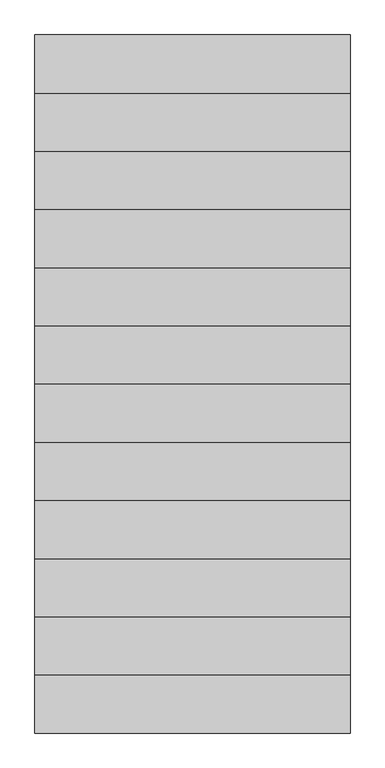
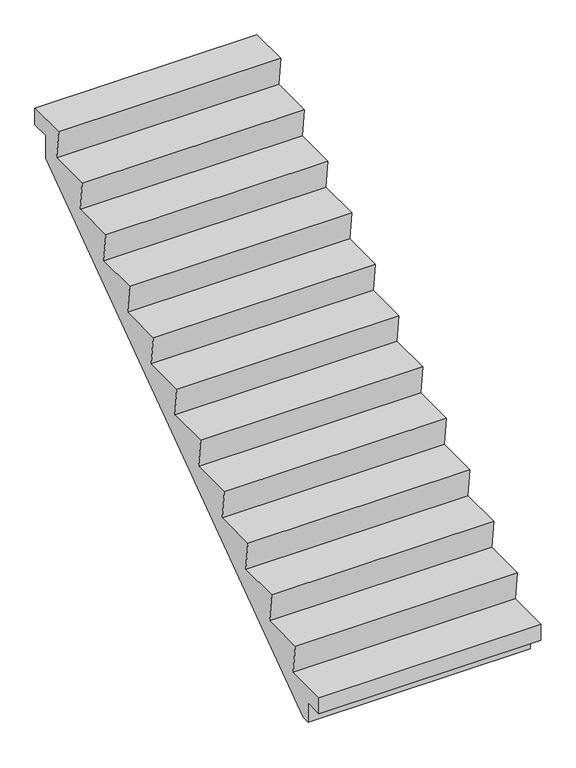
"""IFC4 building model written with IfcOpenShell, lengths in millimetres: stair geometry, NLRS_24_GM_LB_rechte steektrap prefab-AV_gen_rsf : prefab trap_gen__aant=11 b=1200 a=220 o=172.7 zonder bomen."""

from ifc_helpers import new_model, si_unit, frame, origin, place, context, project, spatial, polyline, outline, extrude, source, transform, mapped, element, save


def stair_98d4c19e(model_context):
    return source(origin(), model_context, "Body", "SweptSolid", [
        extrude(outline(polyline([(2400.0, 1900.0), (2640.0, 1900.0), (2640.0, 1800.0), (2530.0, 1800.0), (2530.0, 1658.5925892), (-80.254966, -220.0), (-130.0, -220.0), (-130.0, -100.0), (-240.0, -100.0), (-240.0, 0.0), (20.0, 0.0), (0.0, 172.7272727), (260.0, 172.7272727), (240.0, 345.4545455), (500.0, 345.4545455), (480.0, 518.1818182), (740.0, 518.1818182), (720.0, 690.9090909), (980.0, 690.9090909), (960.0, 863.6363636), (1220.0, 863.6363636), (1200.0, 1036.3636364), (1460.0, 1036.3636364), (1440.0, 1209.0909091), (1700.0, 1209.0909091), (1680.0, 1381.8181818), (1940.0, 1381.8181818), (1920.0, 1554.5454545), (2180.0, 1554.5454545), (2160.0, 1727.2727273), (2420.0, 1727.2727273), (2400.0, 1900.0)])), frame((-650.0, 0.0, 0.0), z_axis=(1.0, 0.0, 0.0), x_axis=(0.0, 1.0, 0.0)), (0.0, 0.0, 1.0), 1300.0),
    ])


if __name__ == "__main__":
    model = new_model("IFC4")
    model_context = context("Model", 3, world=origin())
    ifc_project = project(units=[si_unit("LENGTHUNIT", "METRE", prefix="MILLI")], contexts=[model_context])
    site = spatial("IfcSite", under=ifc_project)
    building = spatial("IfcBuilding", under=site)
    placement = place(None, origin())
    stair_shape = stair_98d4c19e(model_context)
    element("IfcStair", 1, ObjectType="NLRS_24_GM_LB_rechte steektrap prefab-AV_gen_rsf : prefab trap_gen__aant=11 b=1200 a=220 o=172.7 zonder bomen", at=placement, inside=building, context=model_context, shape_type="MappedRepresentation", body=[
        mapped(stair_shape, transform((0.0, 0.0, 0.0), x_axis=(1.0, 0.0, 0.0), y_axis=(0.0, 1.0, 0.0), z_axis=(0.0, 0.0, 1.0))),
    ])
    save(model, "model.ifc")

# Revit data of these elements
# Type "NLRS_24_GM_LB_rechte steektrap prefab-AV_gen_rsf : prefab trap_gen__aant=11 b=1200 a=220 o=172.7 zonder bomen"
#   IfcExportAs = "IfcStair"
#   Type Comments = " "
#   Model = " "
#   Manufacturer = " "
#   Keynote = " "
#   Description = "rechte steektrap prefab\r\naant=11 b=1200 a=220 o=181,8\r\nzonder bomen"
#   Assembly Code = "24.11"
#   Aantrede onder = 240 mm
#   Width = 1300 mm
#   Wel diepte = 20 mm
#   Trapboom breedte = 0 mm
#   Thickness = 120 mm
#   Optrede onderste trede = 220 mm
#   NLRS_C_lengte = 2400 mm
#   Length = 2880 mm
#   Hoogte oplegnok onder = 100 mm
#   Hoogte oplegnok boven = 100 mm
#   Height = 1900 mm
#   Breedte oplegnok boven = 110 mm
#   BottomCalc = 0 mm
#   Actual Tread Depth = 240 mm
#   Actual Riser Height = 172.727 mm
#   Actual Number of Tread = 10
#   Actual Number of Risers = 11
#   Aantrede boven = 240 mm
#   Aantal treden max dertig = 11
#   Trapboom = no
#   Oplegnok onder = yes
#   NLRS_C_materiaal = NLRS_f2_beton prefab_gen_rsf
#   Default Elevation = 0
# Element 1 (IfcStair, "NLRS_24_GM_LB_rechte steektrap prefab-AV_gen_rsf : prefab trap_gen__aant=11 b=1200 a=220 o=172.7 zonder bomen")
#   Materials on its faces: "NLRS_f2_beton prefab_gen_rsf"
# Materials
#   "NLRS_f2_beton prefab_gen_rsf": class "F - Niet gebakken kunststeen", colour RGB 129 133 118, transparency 0, Keynote = "f2", Manufacturer = "Revit Standards Foundation", URL = "www.revitstandards.org", Description = "beton prefab", Cost = 0
